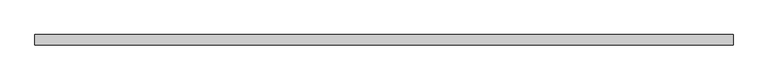
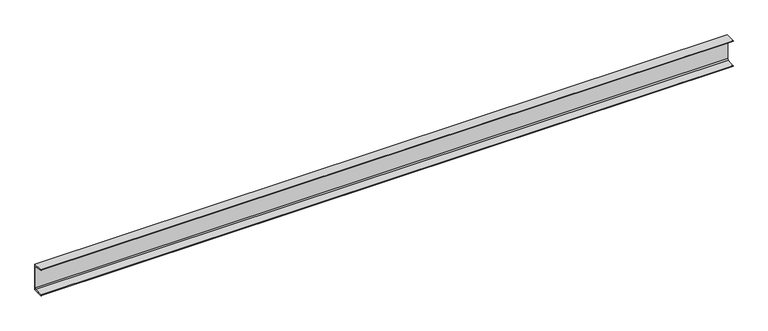
"""IFC4 building model written with IfcOpenShell, lengths in millimetres: beam geometry, C-образный профиль (ГОСТ 8240-89) Балки : [ 22."""

from ifc_helpers import new_model, si_unit, point, frame, frame_2d, origin, place, context, project, spatial, polyline, circle_curve, trimmed, segment, composite_curve, outline, extrude, source, transform, mapped, element, save


def beam_033e1665(model_context):
    return source(origin(), model_context, "Body", "SweptSolid", [
        extrude(outline(composite_curve([segment(polyline([(22.1, 110.0), (22.1, -110.0), (-59.9, -110.0), (-59.9, -108.9686971)]), True, "CONTINUOUS"), segment(trimmed(circle_curve(frame_2d((-55.9, -108.9686971)), 4.0), [point((-59.9, -108.9686971))], [point((-56.3765809, -104.9971897))], False, "CARTESIAN"), True, "CONTINUOUS"), segment(polyline([(-56.3765809, -104.9971897), (7.8914522, -97.2850257)]), True, "CONTINUOUS"), segment(trimmed(circle_curve(frame_2d((6.7, -87.3562574)), 10.0), [point((7.8914522, -97.2850257))], [point((16.7, -87.3562574))], True, "CARTESIAN"), True, "CONTINUOUS"), segment(polyline([(16.7, -87.3562574), (16.7, 87.3562574)]), True, "CONTINUOUS"), segment(trimmed(circle_curve(frame_2d((6.7, 87.3562574)), 10.0), [point((16.7, 87.3562574))], [point((7.8914522, 97.2850257))], True, "CARTESIAN"), True, "CONTINUOUS"), segment(polyline([(7.8914522, 97.2850257), (-56.3765809, 104.9971897)]), True, "CONTINUOUS"), segment(trimmed(circle_curve(frame_2d((-55.9, 108.9686971)), 4.0), [point((-56.3765809, 104.9971897))], [point((-59.9, 108.9686971))], False, "CARTESIAN"), True, "CONTINUOUS"), segment(polyline([(-59.9, 108.9686971), (-59.9, 110.0), (22.1, 110.0)]), True, "CONTINUOUS")], self_intersect=False)), frame((-2802.5, 0.0, 0.0), z_axis=(1.0, 0.0, 0.0), x_axis=(0.0, 1.0, 0.0)), (0.0, 0.0, 1.0), 5605.0),
    ])


if __name__ == "__main__":
    model = new_model("IFC4")
    model_context = context("Model", 3, world=origin())
    ifc_project = project(units=[si_unit("LENGTHUNIT", "METRE", prefix="MILLI")], contexts=[model_context])
    site = spatial("IfcSite", under=ifc_project)
    building = spatial("IfcBuilding", under=site)
    placement = place(None, origin())
    beam_shape = beam_033e1665(model_context)
    element("IfcBeam", 1, ObjectType="C-образный профиль (ГОСТ 8240-89) Балки : [ 22", at=placement, inside=building, context=model_context, shape_type="MappedRepresentation", body=[
        mapped(beam_shape, transform((0.0, 0.0, 0.0), x_axis=(1.0, 0.0, 0.0), y_axis=(0.0, 1.0, 0.0), z_axis=(0.0, 0.0, 1.0))),
    ])
    save(model, "model.ifc")

# Revit data of these elements
# Type "C-образный профиль (ГОСТ 8240-89) Балки : [ 22"
#   tf = 9.5 mm
#   ri = 4 mm
#   ra = 10 mm
#   W = 0.20594
#   Vz = 110 mm
#   Vy = 59.9 mm
#   Vpz = 110 mm
#   Vpy = 22.1 mm
#   Уклон = 0.12
#   Length [instance default] = 1500 mm
#   bf = 82 mm
#   d = 220 mm
#   tw = 5.4 mm
#   A = 0.00267 m²
#   Structural Material [instance default] = Металл - Сталь - 345 МПa
#   Assembly Code = ""
# Element 1 (IfcBeam, "C-образный профиль (ГОСТ 8240-89) Балки : [ 22")
#   Structural Material = C235
#   Materials on its faces: "C235"
# Materials
#   "Металл - Сталь - 345 МПa": class "Металл", colour RGB 247 247 247, transparency 0
#   "C235": class "Не назначено", colour RGB 0 0 0, transparency 0
